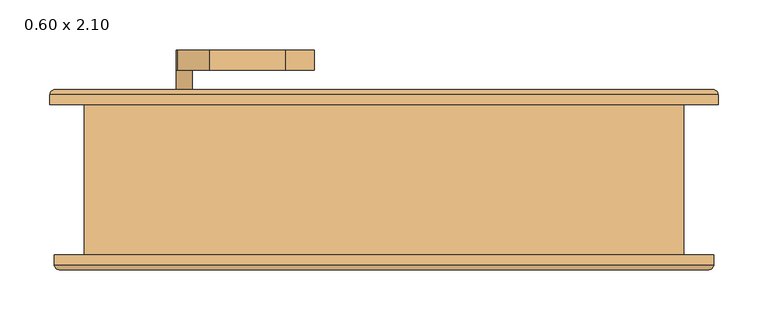
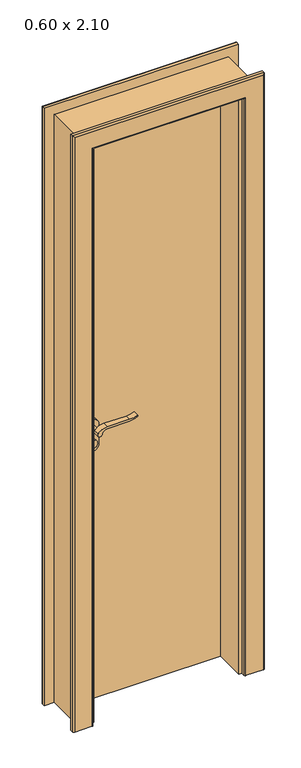
"""IFC4 building model written with IfcOpenShell, lengths in millimetres: door geometry, PORTA_DE_ABRIR_MADEIRA : 0.60 x 2.10."""

import ifcopenshell
import ifcopenshell.guid

model = None  # the IFC model being written
_history = None  # IfcOwnerHistory: only IFC2X3 demands one
_inside = {}  # id of a spatial element -> (the spatial element, [elements in it])
_under = {}  # id of a project, library or spatial element -> (it, [spatial elements below it])
_declared = {}  # id of a project -> (the project, [libraries it declares])
_typed = {}  # id of a type object -> (the type object, [elements of that type])
_made_of = {}  # id of a material, layer set ... -> (it, [elements and type objects made of it])


def new_model(schema):
    """Start an empty IFC model of exactly this schema.

    Asked for "IFC4X3", IfcOpenShell would pick the latest addendum, in which some entities
    have other attributes; the version numbers below select the first issue.
    IFC2X3 requires an IfcOwnerHistory on every rooted entity: one is made here for all.
    """
    global model, _history
    if schema == "IFC4X3":
        model = ifcopenshell.file(schema_version=(4, 3, 0, 0))
    else:
        model = ifcopenshell.file(schema=schema)
    _inside.clear()
    _under.clear()
    _declared.clear()
    _typed.clear()
    _made_of.clear()
    _history = None
    if model.schema == "IFC2X3":
        org = make("IfcOrganization", Name="unknown")
        user = make(
            "IfcPersonAndOrganization",
            ThePerson=make("IfcPerson", FamilyName="unknown"),
            TheOrganization=org,
        )
        app = make(
            "IfcApplication",
            ApplicationDeveloper=org,
            Version="unknown",
            ApplicationFullName="unknown",
            ApplicationIdentifier="unknown",
        )
        _history = make(
            "IfcOwnerHistory",
            OwningUser=user,
            OwningApplication=app,
            ChangeAction="ADDED",
            CreationDate=0,
        )
    return model


def make(cls, **values):
    """One entity of the class cls with the attributes given. An attribute that is None is left unset."""
    return model.create_entity(
        cls, **{name: value for name, value in values.items() if value is not None}
    )


def rooted(cls, **values):
    """An entity with a GlobalId (a new one), such as an element, a storey or a relation."""
    return make(cls, GlobalId=ifcopenshell.guid.new(), OwnerHistory=_history, **values)


def si_unit(unit_type, name, prefix=None):
    """IfcSIUnit, for example si_unit("LENGTHUNIT", "METRE", prefix="MILLI")."""
    return make("IfcSIUnit", UnitType=unit_type, Prefix=prefix, Name=name)


def assignment(units):
    """IfcUnitAssignment: the units of a project."""
    return None if units is None else make("IfcUnitAssignment", Units=units)


def point(xyz):
    """IfcCartesianPoint."""
    return None if xyz is None else make("IfcCartesianPoint", Coordinates=xyz)


def direction(xyz):
    """IfcDirection."""
    return None if xyz is None else make("IfcDirection", DirectionRatios=xyz)


def frame(location, z_axis=None, x_axis=None):
    """IfcAxis2Placement3D, a coordinate frame: its origin and axes. An axis left out is left unset."""
    return make(
        "IfcAxis2Placement3D",
        Location=point(location),
        Axis=direction(z_axis),
        RefDirection=direction(x_axis),
    )


def frame_2d(location, x_axis=None):
    """IfcAxis2Placement2D, a coordinate frame in the plane: its origin and x axis."""
    return make(
        "IfcAxis2Placement2D", Location=point(location), RefDirection=direction(x_axis)
    )


def origin():
    """The frame at (0, 0, 0) with its axes left unset."""
    return frame((0.0, 0.0, 0.0))


def origin_with_axes():
    """The frame at (0, 0, 0) with the z axis (0, 0, 1) and the x axis (1, 0, 0) written out."""
    return frame((0.0, 0.0, 0.0), z_axis=(0.0, 0.0, 1.0), x_axis=(1.0, 0.0, 0.0))


def place(relative_to, where):
    """IfcLocalPlacement: puts the frame where relative to a parent placement (None: the world)."""
    return make(
        "IfcLocalPlacement", PlacementRelTo=relative_to, RelativePlacement=where
    )


def context(
    kind, dimensions, precision=None, world=None, true_north=None, identifier=None
):
    """IfcGeometricRepresentationContext, for example the 3D "Model" context."""
    return make(
        "IfcGeometricRepresentationContext",
        ContextIdentifier=identifier,
        ContextType=kind,
        CoordinateSpaceDimension=dimensions,
        Precision=precision,
        WorldCoordinateSystem=world,
        TrueNorth=true_north,
    )


def project(units=None, contexts=None):
    """IfcProject with its units and contexts."""
    return rooted(
        "IfcProject",
        Name="project",
        RepresentationContexts=contexts,
        UnitsInContext=assignment(units),
    )


def spatial(cls, under=None, at=None, **own):
    """A site, building, storey or space (cls), placed at a placement, below another one or the project."""
    s = rooted(cls, ObjectPlacement=at, **own)
    if under is not None:
        _under.setdefault(under.id(), (under, []))[1].append(s)
    return s


def polyline(points):
    """IfcPolyline through the points."""
    return make("IfcPolyline", Points=[point(p) for p in points])


def circle_curve(where, radius):
    """IfcCircle in the frame where."""
    return make("IfcCircle", Position=where, Radius=radius)


def ellipse_curve(where, semi_axis1, semi_axis2):
    """IfcEllipse in the frame where."""
    return make(
        "IfcEllipse", Position=where, SemiAxis1=semi_axis1, SemiAxis2=semi_axis2
    )


def trimmed(basis, trim1, trim2, sense, master):
    """IfcTrimmedCurve: the piece of a basis curve between two trims."""
    return make(
        "IfcTrimmedCurve",
        BasisCurve=basis,
        Trim1=trim1,
        Trim2=trim2,
        SenseAgreement=sense,
        MasterRepresentation=master,
    )


def segment(curve, same_sense, transition):
    """IfcCompositeCurveSegment."""
    return make(
        "IfcCompositeCurveSegment",
        Transition=transition,
        SameSense=same_sense,
        ParentCurve=curve,
    )


def composite_curve(segments, self_intersect=None):
    """IfcCompositeCurve: segments joined end to end."""
    return make("IfcCompositeCurve", Segments=segments, SelfIntersect=self_intersect)


def outline(outer, holes=None, kind="AREA"):
    """IfcArbitraryClosedProfileDef: a profile drawn as a closed curve; with holes, ...WithVoids."""
    if holes is None:
        return make("IfcArbitraryClosedProfileDef", ProfileType=kind, OuterCurve=outer)
    return make(
        "IfcArbitraryProfileDefWithVoids",
        ProfileType=kind,
        OuterCurve=outer,
        InnerCurves=holes,
    )


def extrude(swept, where, along, depth):
    """IfcExtrudedAreaSolid: the profile swept, set in the frame where, extruded along a direction by depth."""
    return make(
        "IfcExtrudedAreaSolid",
        SweptArea=swept,
        Position=where,
        ExtrudedDirection=direction(along),
        Depth=depth,
    )


def faces_of(points, faces, orient=None, outer=None):
    """IfcFace entities. A face is a list of loops; a loop is a list of indices into points, from 0.

    orient and outer hold one flag for each loop. By default every Orientation is true, the
    first loop of a face is its IfcFaceOuterBound and the others are IfcFaceBound.
    """
    made = []
    for i, loops in enumerate(faces):
        bounds = []
        for j, loop in enumerate(loops):
            is_outer = j == 0 if outer is None else outer[i][j]
            bounds.append(
                make(
                    "IfcFaceOuterBound" if is_outer else "IfcFaceBound",
                    Bound=make("IfcPolyLoop", Polygon=[points[k] for k in loop]),
                    Orientation=True if orient is None else orient[i][j],
                )
            )
        made.append(make("IfcFace", Bounds=bounds))
    return made


def faceted_brep(points, faces, orient=None, outer=None, voids=None):
    """IfcFacetedBrep: a solid bounded by flat faces; with voids (closed shells), ...WithVoids."""
    shared = [point(p) for p in points]
    hull = make("IfcClosedShell", CfsFaces=faces_of(shared, faces, orient, outer))
    if voids is None:
        return make("IfcFacetedBrep", Outer=hull)
    return make(
        "IfcFacetedBrepWithVoids",
        Outer=hull,
        Voids=[
            make(cls, CfsFaces=faces_of(shared, fs, o, b)) for cls, fs, o, b in voids
        ],
    )


def shape(context_of_items, identifier, shape_type, items):
    """IfcShapeRepresentation: the items that make up one representation, for example the "Body"."""
    return make(
        "IfcShapeRepresentation",
        ContextOfItems=context_of_items,
        RepresentationIdentifier=identifier,
        RepresentationType=shape_type,
        Items=items,
    )


def source(mapping_origin, context_of_items, identifier, shape_type, items):
    """IfcRepresentationMap: a shape defined once, which mapped items show again and again."""
    return make(
        "IfcRepresentationMap",
        MappingOrigin=mapping_origin,
        MappedRepresentation=shape(context_of_items, identifier, shape_type, items),
    )


def transform(
    local_origin,
    x_axis=None,
    y_axis=None,
    z_axis=None,
    scale=None,
    scale2=None,
    scale3=None,
    uniform=True,
):
    """IfcCartesianTransformationOperator3D, or its non-uniform kind. x_axis, y_axis, z_axis: its Axis1, 2, 3."""
    if uniform:
        return make(
            "IfcCartesianTransformationOperator3D",
            Axis1=direction(x_axis),
            Axis2=direction(y_axis),
            LocalOrigin=point(local_origin),
            Scale=scale,
            Axis3=direction(z_axis),
        )
    return make(
        "IfcCartesianTransformationOperator3DnonUniform",
        Axis1=direction(x_axis),
        Axis2=direction(y_axis),
        LocalOrigin=point(local_origin),
        Scale=scale,
        Axis3=direction(z_axis),
        Scale2=scale2,
        Scale3=scale3,
    )


def mapped(mapping_source, mapping_target):
    """IfcMappedItem: shows the shape of a source again, moved by a transform."""
    return make(
        "IfcMappedItem", MappingSource=mapping_source, MappingTarget=mapping_target
    )


def made_of(thing, what):
    """Note that an element or type object is made of a material, layer set ...; save() writes the relation."""
    if what is not None:
        _made_of.setdefault(what.id(), (what, []))[1].append(thing)
    return thing


def element(
    cls,
    number,
    at=None,
    inside=None,
    cuts=None,
    type_object=None,
    material=None,
    context=None,
    identifier="Body",
    shape_type=None,
    held_by="IfcProductDefinitionShape",
    body=None,
    shapes=None,
    **own,
):
    """One element of the class cls, such as IfcWall. Its Tag is "e" and its number.

    at: its placement. inside: the storey or other place that contains it. cuts: it is an
    opening in that element (IfcRelVoidsElement). A single representation is given by context,
    identifier, shape_type and body (its items); several are given by shapes. held_by: the class
    of the entity that holds the representations. save() writes the other relations.
    """
    e = rooted(cls, Tag="e%d" % number, ObjectPlacement=at, **own)
    if body is not None:
        shapes = [shape(context, identifier, shape_type, body)]
    if shapes is not None:
        e.Representation = make(held_by, Representations=shapes)
    if inside is not None:
        _inside.setdefault(inside.id(), (inside, []))[1].append(e)
    if cuts is not None:
        rooted(
            "IfcRelVoidsElement", RelatingBuildingElement=cuts, RelatedOpeningElement=e
        )
    if type_object is not None:
        _typed.setdefault(type_object.id(), (type_object, []))[1].append(e)
    return made_of(e, material)


def aggregate(whole, parts):
    """IfcRelAggregates: a whole, such as a stair, and the parts it consists of."""
    return rooted("IfcRelAggregates", RelatingObject=whole, RelatedObjects=parts)


def save(model, path):
    """Write the relations noted so far, then the file.

    IfcRelAggregates (storeys below a building ...), IfcRelContainedInSpatialStructure (elements
    in a storey), IfcRelDefinesByType, IfcRelAssociatesMaterial and IfcRelDeclares: one each for
    every whole, place, type object, material and project.
    """
    for whole, parts in _under.values():
        aggregate(whole, parts)
    for where, things in _inside.values():
        rooted(
            "IfcRelContainedInSpatialStructure",
            RelatedElements=things,
            RelatingStructure=where,
        )
    for kind, things in _typed.values():
        rooted("IfcRelDefinesByType", RelatedObjects=things, RelatingType=kind)
    for what, things in _made_of.values():
        rooted("IfcRelAssociatesMaterial", RelatedObjects=things, RelatingMaterial=what)
    for by, libraries in _declared.values():
        rooted("IfcRelDeclares", RelatingContext=by, RelatedDefinitions=libraries)
    model.write(path)


def plane_surface(at):
    """IfcPlane: the flat surface through the origin of the frame at, square to its z axis."""
    return make("IfcPlane", Position=at)


def cylinder_surface(at, radius):
    """IfcCylindricalSurface: all points at the distance radius from the z axis of the frame at."""
    return make("IfcCylindricalSurface", Position=at, Radius=radius)


def advanced_brep(points, edges, surfaces, faces):
    """IfcAdvancedBrep: a solid bounded by faces that lie on surfaces and meet in shared edges.

    An edge is (start, end): straight between two places in points (the first is 0);
    or (start, end, curve); or (start, end, curve, False) where it runs against its curve.
    A face is (place in surfaces, loops), or (place, loops, False) where it looks against
    its surface's normal. A loop lists edges by number (the first is 1), with a minus sign
    where the edge is run from its end to its start. The first loop is the outer one.
    """
    corners = [point(p) for p in points]
    vertices = [make("IfcVertexPoint", VertexGeometry=c) for c in corners]
    made = []
    for start, end, *more in edges:
        made.append(
            make(
                "IfcEdgeCurve",
                EdgeStart=vertices[start],
                EdgeEnd=vertices[end],
                EdgeGeometry=more[0] if more else make("IfcPolyline", Points=[corners[start], corners[end]]),
                SameSense=more[1] if len(more) > 1 else True,
            )
        )
    hull = []
    for where, loops, *sense in faces:
        bounds = []
        for j, loop in enumerate(loops):
            ring = [make("IfcOrientedEdge", EdgeElement=made[abs(k) - 1], Orientation=k > 0) for k in loop]
            bounds.append(
                make(
                    "IfcFaceOuterBound" if j == 0 else "IfcFaceBound",
                    Bound=make("IfcEdgeLoop", EdgeList=ring),
                    Orientation=True,
                )
            )
        hull.append(make("IfcAdvancedFace", Bounds=bounds, FaceSurface=surfaces[where], SameSense=sense[0] if sense else True))
    return make("IfcAdvancedBrep", Outer=make("IfcClosedShell", CfsFaces=hull))


def door_0_60_x_2_10_4441030f(model_context):
    return source(origin(), model_context, "Body", "SolidModel", [
        extrude(outline(composite_curve([segment(trimmed(circle_curve(frame_2d((940.0, -200.0)), 15.0), [point((940.0, -185.0))], [point((940.0, -215.0))], False, "CARTESIAN"), True, "CONTINUOUS"), segment(trimmed(circle_curve(frame_2d((940.0, -200.0)), 15.0), [point((940.0, -215.0))], [point((940.0, -185.0))], False, "CARTESIAN"), True, "CONTINUOUS")], self_intersect=False)), frame((0.0, 15.0, 0.0), z_axis=(0.0, 1.0, 0.0), x_axis=(0.0, 0.0, 1.0)), (0.0, 0.0, 1.0), 10.0),
        extrude(outline(composite_curve([segment(trimmed(circle_curve(frame_2d((940.0, -200.0)), 15.0), [point((940.0, -185.0))], [point((940.0, -215.0))], False, "CARTESIAN"), True, "CONTINUOUS"), segment(trimmed(circle_curve(frame_2d((940.0, -200.0)), 15.0), [point((940.0, -215.0))], [point((940.0, -185.0))], False, "CARTESIAN"), True, "CONTINUOUS")], self_intersect=False)), frame((0.0, 80.0, 0.0), z_axis=(0.0, 1.0, 0.0), x_axis=(0.0, 0.0, 1.0)), (0.0, 0.0, 1.0), 10.0),
        extrude(outline(composite_curve([segment(trimmed(circle_curve(frame_2d((1000.0, -200.0)), 8.0), [point((1004.6523287, -206.5081363))], [point((1000.0, -192.0))], False, "CARTESIAN"), True, "CONTINUOUS"), segment(trimmed(circle_curve(frame_2d((994.8738613, -174.6138099)), 18.1261387), [point((1000.0, -192.0))], [point((1013.0, -174.6138099))], True, "CARTESIAN"), True, "CONTINUOUS"), segment(polyline([(1013.0, -174.6138099), (1013.0, -98.3564091)]), True, "CONTINUOUS"), segment(trimmed(circle_curve(frame_2d((1072.2709207, -101.9396612)), 59.3791355), [point((1013.0, -98.3564091))], [point((1022.2135558, -70.0))], False, "CARTESIAN"), True, "CONTINUOUS"), segment(polyline([(1022.2135558, -70.0), (1025.0, -70.0)]), True, "CONTINUOUS"), segment(trimmed(circle_curve(frame_2d((1103.2850638, -98.4227909)), 83.2850902), [point((1025.0, -70.0))], [point((1020.0, -98.3564091))], True, "CARTESIAN"), True, "CONTINUOUS"), segment(polyline([(1020.0, -98.3564091), (1020.0, -174.6325667)]), True, "CONTINUOUS"), segment(trimmed(circle_curve(frame_2d((982.7555521, -176.3324871)), 37.2832219), [point((1020.0, -174.6325667))], [point((1004.6523287, -206.5081363))], False, "CARTESIAN"), True, "CONTINUOUS")], self_intersect=False)), frame((0.0, -25.0, 0.0), z_axis=(0.0, 1.0, 0.0), x_axis=(0.0, 0.0, 1.0)), (0.0, 0.0, 1.0), 20.0),
        extrude(outline(composite_curve([segment(trimmed(circle_curve(frame_2d((994.8738682, -174.6138122)), 18.1261318), [point((999.9999903, -192.0))], [point((1013.0, -174.6138122))], True, "CARTESIAN"), True, "CONTINUOUS"), segment(polyline([(1013.0, -174.6138122), (1013.0, -98.3564091)]), True, "CONTINUOUS"), segment(trimmed(circle_curve(frame_2d((1072.2709207, -101.9396612)), 59.3791355), [point((1013.0, -98.3564091))], [point((1022.2135558, -70.0))], False, "CARTESIAN"), True, "CONTINUOUS"), segment(polyline([(1022.2135558, -70.0), (1025.0, -70.0)]), True, "CONTINUOUS"), segment(trimmed(circle_curve(frame_2d((1103.2850638, -98.4227909)), 83.2850902), [point((1025.0, -70.0))], [point((1020.0, -98.3564091))], True, "CARTESIAN"), True, "CONTINUOUS"), segment(polyline([(1020.0, -98.3564091), (1020.0, -174.6325667)]), True, "CONTINUOUS"), segment(trimmed(circle_curve(frame_2d((982.7555521, -176.3324871)), 37.2832219), [point((1020.0, -174.6325667))], [point((1004.6523287, -206.5081363))], False, "CARTESIAN"), True, "CONTINUOUS"), segment(trimmed(circle_curve(frame_2d((1000.0, -200.0)), 8.0), [point((1004.6523287, -206.5081363))], [point((999.9999903, -192.0))], False, "CARTESIAN"), True, "CONTINUOUS")], self_intersect=False)), frame((0.0, 110.0, 0.0), z_axis=(0.0, 1.0, 0.0), x_axis=(0.0, 0.0, 1.0)), (0.0, 0.0, 1.0), 20.0),
        extrude(outline(composite_curve([segment(trimmed(circle_curve(frame_2d((1000.0, -200.0)), 8.0), [point((1000.0, -192.0))], [point((1000.0, -208.0))], False, "CARTESIAN"), True, "CONTINUOUS"), segment(trimmed(circle_curve(frame_2d((1000.0, -200.0)), 8.0), [point((1000.0, -208.0))], [point((1000.0, -192.0))], False, "CARTESIAN"), True, "CONTINUOUS")], self_intersect=False)), frame((0.0, -5.0, 0.0), z_axis=(0.0, 1.0, 0.0), x_axis=(0.0, 0.0, 1.0)), (0.0, 0.0, 1.0), 30.0),
        extrude(outline(composite_curve([segment(trimmed(circle_curve(frame_2d((1000.0, -200.0)), 8.0), [point((1000.0, -192.0))], [point((1000.0, -208.0))], False, "CARTESIAN"), True, "CONTINUOUS"), segment(trimmed(circle_curve(frame_2d((1000.0, -200.0)), 8.0), [point((1000.0, -208.0))], [point((1000.0, -192.0))], False, "CARTESIAN"), True, "CONTINUOUS")], self_intersect=False)), frame((0.0, 80.0, 0.0), z_axis=(0.0, 1.0, 0.0), x_axis=(0.0, 0.0, 1.0)), (0.0, 0.0, 1.0), 30.0),
        extrude(outline(composite_curve([segment(trimmed(circle_curve(frame_2d((930.0, -200.0)), 25.0), [point((930.0, -225.0))], [point((930.0, -175.0))], False, "CARTESIAN"), True, "CONTINUOUS"), segment(polyline([(930.0, -175.0), (1000.0, -175.0)]), True, "CONTINUOUS"), segment(trimmed(circle_curve(frame_2d((1000.0, -200.0)), 25.0), [point((1000.0, -175.0))], [point((1000.0, -225.0))], False, "CARTESIAN"), True, "CONTINUOUS"), segment(polyline([(1000.0, -225.0), (930.0, -225.0)]), True, "CONTINUOUS")], self_intersect=False)), frame((0.0, 25.0, 0.0), z_axis=(0.0, 1.0, 0.0), x_axis=(0.0, 0.0, 1.0)), (0.0, 0.0, 1.0), 10.0),
        extrude(outline(composite_curve([segment(trimmed(circle_curve(frame_2d((930.0, -200.0)), 25.0), [point((930.0, -225.0))], [point((930.0, -175.0))], False, "CARTESIAN"), True, "CONTINUOUS"), segment(polyline([(930.0, -175.0), (1000.0, -175.0)]), True, "CONTINUOUS"), segment(trimmed(circle_curve(frame_2d((1000.0, -200.0)), 25.0), [point((1000.0, -175.0))], [point((1000.0, -225.0))], False, "CARTESIAN"), True, "CONTINUOUS"), segment(polyline([(1000.0, -225.0), (930.0, -225.0)]), True, "CONTINUOUS")], self_intersect=False)), frame((0.0, 70.0, 0.0), z_axis=(0.0, 1.0, 0.0), x_axis=(0.0, 0.0, 1.0)), (0.0, 0.0, 1.0), 10.0),
        faceted_brep([(-260.0, 35.0, 0.0), (-250.0, 35.0, 0.0), (-250.0, -75.0, 0.0), (-300.0, -75.0, 0.0), (-300.0, 75.0, 0.0), (-260.0, 75.0, 0.0), (-260.0, 75.0, 2100.0), (-260.0, 35.0, 2100.0), (-300.0, 75.0, 2140.0), (300.0, 75.0, 2140.0), (300.0, 75.0, 0.0), (260.0, 75.0, 0.0), (260.0, 75.0, 2100.0), (-300.0, -75.0, 2140.0), (-250.0, -75.0, 2090.0), (250.0, -75.0, 2090.0), (250.0, -75.0, 0.0), (300.0, -75.0, 0.0), (300.0, -75.0, 2140.0), (-250.0, 35.0, 2090.0), (260.0, 35.0, 2100.0), (260.0, 35.0, 0.0), (250.0, 35.0, 0.0), (250.0, 35.0, 2090.0)], [[[0, 1, 2, 3, 4, 5]], [[5, 6, 7, 0]], [[4, 8, 9, 10, 11, 12, 6, 5]], [[3, 13, 8, 4]], [[2, 14, 15, 16, 17, 18, 13, 3]], [[1, 19, 14, 2]], [[0, 7, 20, 21, 22, 23, 19, 1]], [[23, 22, 16, 15]], [[21, 11, 10, 17, 16, 22]], [[12, 11, 21, 20]], [[18, 17, 10, 9]], [[13, 18, 9, 8]], [[19, 23, 15, 14]], [[6, 12, 20, 7]]]),
        advanced_brep(
        [(-330.0, -75.3, 0.0), (-260.0, -75.3, 0.0), (-260.0, -85.3, 0.0), (-265.0, -90.3, 0.0), (-325.0, -90.3, 0.0), (-330.0, -85.3, 0.0), (-330.0, -85.3, 2170.0), (-330.0, -75.3, 2170.0), (-325.0, -90.3, 2165.0), (-265.0, -90.3, 2105.0), (265.0, -90.3, 2105.0), (265.0, -90.3, 0.0), (325.0, -90.3, 0.0), (325.0, -90.3, 2165.0), (-260.0, -85.3, 2100.0), (-260.0, -75.3, 2100.0), (330.0, -75.3, 2170.0), (330.0, -75.3, 0.0), (260.0, -75.3, 0.0), (260.0, -75.3, 2100.0), (330.0, -85.3, 0.0), (260.0, -85.3, 0.0), (260.0, -85.3, 2100.0), (330.0, -85.3, 2170.0)],
        [
            (0, 1),
            (1, 2),
            (2, 3, circle_curve(frame((-265.0, -85.3, 0.0), z_axis=(0.0, 0.0, -1.0), x_axis=(-1.0, 0.0, 0.0)), 5.0)),
            (3, 4),
            (4, 5, circle_curve(frame((-325.0, -85.3, 0.0), z_axis=(0.0, 0.0, -1.0), x_axis=(-1.0, 0.0, 0.0)), 5.0)),
            (5, 0),
            (5, 6),
            (6, 7),
            (7, 0),
            (4, 8),
            (8, 6, ellipse_curve(frame((-325.0, -85.3, 2165.0), z_axis=(-0.7071067811865475, 0.0, -0.7071067811865475), x_axis=(0.7071067811865474, 0.0, -0.7071067811865476)), 7.0710678, 5.0)),
            (3, 9),
            (9, 10),
            (10, 11),
            (11, 12),
            (12, 13),
            (13, 8),
            (2, 14),
            (14, 9, ellipse_curve(frame((-265.0, -85.3, 2105.0), z_axis=(-0.7071067811865475, 0.0, -0.7071067811865475), x_axis=(0.7071067811865474, 0.0, -0.7071067811865476)), 7.0710678, 5.0)),
            (1, 15),
            (15, 14),
            (7, 16),
            (16, 17),
            (17, 18),
            (18, 19),
            (19, 15),
            (17, 20),
            (20, 12, circle_curve(frame((325.0, -85.3, 0.0), z_axis=(0.0, 0.0, -1.0), x_axis=(1.0, 0.0, 0.0)), 5.0)),
            (11, 21, circle_curve(frame((265.0, -85.3, 0.0), z_axis=(0.0, 0.0, -1.0), x_axis=(1.0, 0.0, 0.0)), 5.0)),
            (21, 18),
            (21, 22),
            (22, 19),
            (10, 22, ellipse_curve(frame((265.0, -85.3, 2105.0), z_axis=(0.7071067811865475, 0.0, -0.7071067811865475), x_axis=(0.7071067811865474, 0.0, 0.7071067811865476)), 7.0710678, 5.0)),
            (20, 23),
            (23, 13, ellipse_curve(frame((325.0, -85.3, 2165.0), z_axis=(0.7071067811865475, 0.0, -0.7071067811865475), x_axis=(0.7071067811865474, 0.0, 0.7071067811865476)), 7.0710678, 5.0)),
            (16, 23),
            (6, 23),
            (22, 14),
        ],
        [
            plane_surface(frame((-300.0, 75.0, 0.0), z_axis=(0.0, 0.0, -1.0), x_axis=(0.0, 1.0, 0.0))),
            plane_surface(frame((-330.0, -75.3, 0.0), z_axis=(-1.0, 0.0, 0.0), x_axis=(0.0, 0.0, 1.0))),
            cylinder_surface(frame((-325.0, -85.3, 0.0), z_axis=(0.0, 0.0, -1.0), x_axis=(-1.0, 0.0, 0.0)), 5.0),
            plane_surface(frame((-325.0, -90.3, 0.0), z_axis=(0.0, -1.0, 0.0), x_axis=(0.0, 0.0, 1.0))),
            cylinder_surface(frame((-265.0, -85.3, 0.0), z_axis=(0.0, 0.0, -1.0), x_axis=(-1.0, 0.0, 0.0)), 5.0),
            plane_surface(frame((-260.0, -85.3, 0.0), z_axis=(1.0, 0.0, 0.0), x_axis=(0.0, 0.0, 1.0))),
            plane_surface(frame((-260.0, -75.3, 0.0), z_axis=(0.0, 1.0, 0.0), x_axis=(0.0, 0.0, 1.0))),
            plane_surface(frame((300.0, 75.0, 0.0), z_axis=(0.0, 0.0, -1.0), x_axis=(0.0, 1.0, 0.0))),
            plane_surface(frame((260.0, -85.3, 2100.0), z_axis=(-1.0, 0.0, 0.0), x_axis=(0.0, 0.0, -1.0))),
            cylinder_surface(frame((265.0, -85.3, 2140.0), z_axis=(0.0, 0.0, 1.0), x_axis=(1.0, 0.0, 0.0)), 5.0),
            cylinder_surface(frame((325.0, -85.3, 2140.0), z_axis=(0.0, 0.0, 1.0), x_axis=(1.0, 0.0, 0.0)), 5.0),
            plane_surface(frame((330.0, -75.3, 2170.0), z_axis=(1.0, 0.0, 0.0), x_axis=(0.0, 0.0, -1.0))),
            plane_surface(frame((-330.0, -75.3, 2170.0), z_axis=(0.0, 0.0, 1.0), x_axis=(1.0, 0.0, 0.0))),
            plane_surface(frame((-260.0, -85.3, 2100.0), z_axis=(0.0, 0.0, -1.0), x_axis=(1.0, 0.0, 0.0))),
            cylinder_surface(frame((-300.0, -85.3, 2165.0), z_axis=(-1.0, 0.0, 0.0), x_axis=(0.0, 0.0, 1.0)), 5.0),
            cylinder_surface(frame((-300.0, -85.3, 2105.0), z_axis=(-1.0, 0.0, 0.0), x_axis=(0.0, 0.0, 1.0)), 5.0),
        ],
        [
            (0, [[1, 2, 3, 4, 5, 6]]),
            (1, [[7, 8, 9, -6]]),
            (2, [[10, 11, -7, -5]]),
            (3, [[12, 13, 14, 15, 16, 17, -10, -4]]),
            (4, [[18, 19, -12, -3]]),
            (5, [[20, 21, -18, -2]]),
            (6, [[-9, 22, 23, 24, 25, 26, -20, -1]]),
            (7, [[27, 28, -15, 29, 30, -24]]),
            (8, [[-25, -30, 31, 32]]),
            (9, [[-31, -29, -14, 33]]),
            (10, [[-16, -28, 34, 35]]),
            (11, [[-34, -27, -23, 36]]),
            (12, [[37, -36, -22, -8]]),
            (13, [[-26, -32, 38, -21]]),
            (14, [[-17, -35, -37, -11]]),
            (15, [[-38, -33, -13, -19]]),
        ],
    ),
        advanced_brep(
        [(-329.3155593, 90.2647517, 0.0), (-269.3155593, 90.2647517, 0.0), (-264.3155593, 85.2647517, 0.0), (-264.3155593, 75.2647517, 0.0), (-334.3155593, 75.2647517, 0.0), (-334.3155593, 85.2647517, 0.0), (-334.3155593, 85.2647517, 2174.3155593), (-329.3155593, 90.2647517, 2169.3155593), (-334.3155593, 75.2647517, 2174.3155593), (-264.3155593, 75.2647517, 2104.3155593), (264.3155593, 75.2647517, 2104.3155593), (264.3155593, 75.2647517, 0.0), (334.3155593, 75.2647517, 0.0), (334.3155593, 75.2647517, 2174.3155593), (-264.3155593, 85.2647517, 2104.3155593), (-269.3155593, 90.2647517, 2109.3155593), (329.3155593, 90.2647517, 2169.3155593), (329.3155593, 90.2647517, 0.0), (269.3155593, 90.2647517, 0.0), (269.3155593, 90.2647517, 2109.3155593), (334.3155593, 85.2647517, 0.0), (264.3155593, 85.2647517, 0.0), (264.3155593, 85.2647517, 2104.3155593), (334.3155593, 85.2647517, 2174.3155593)],
        [
            (0, 1),
            (1, 2, circle_curve(frame((-269.3155593, 85.2647517, 0.0), z_axis=(0.0, 0.0, -1.0), x_axis=(-1.0, 0.0, 0.0)), 5.0)),
            (2, 3),
            (3, 4),
            (4, 5),
            (5, 0, circle_curve(frame((-329.3155593, 85.2647517, 0.0), z_axis=(0.0, 0.0, -1.0), x_axis=(-1.0, 0.0, 0.0)), 5.0)),
            (5, 6),
            (6, 7, ellipse_curve(frame((-329.3155593, 85.2647517, 2169.3155593), z_axis=(-0.7071067811865475, 0.0, -0.7071067811865475), x_axis=(0.7071067811865474, 0.0, -0.7071067811865476)), 7.0710678, 5.0)),
            (7, 0),
            (4, 8),
            (8, 6),
            (3, 9),
            (9, 10),
            (10, 11),
            (11, 12),
            (12, 13),
            (13, 8),
            (2, 14),
            (14, 9),
            (1, 15),
            (15, 14, ellipse_curve(frame((-269.3155593, 85.2647517, 2109.3155593), z_axis=(-0.7071067811865475, 0.0, -0.7071067811865475), x_axis=(0.7071067811865474, 0.0, -0.7071067811865476)), 7.0710678, 5.0)),
            (7, 16),
            (16, 17),
            (17, 18),
            (18, 19),
            (19, 15),
            (17, 20, circle_curve(frame((329.3155593, 85.2647517, 0.0), z_axis=(0.0, 0.0, -1.0), x_axis=(1.0, 0.0, 0.0)), 5.0)),
            (20, 12),
            (11, 21),
            (21, 18, circle_curve(frame((269.3155593, 85.2647517, 0.0), z_axis=(0.0, 0.0, -1.0), x_axis=(1.0, 0.0, 0.0)), 5.0)),
            (21, 22),
            (22, 19, ellipse_curve(frame((269.3155593, 85.2647517, 2109.3155593), z_axis=(0.7071067811865475, 0.0, -0.7071067811865475), x_axis=(0.7071067811865474, 0.0, 0.7071067811865476)), 7.0710678, 5.0)),
            (10, 22),
            (20, 23),
            (23, 13),
            (16, 23, ellipse_curve(frame((329.3155593, 85.2647517, 2169.3155593), z_axis=(0.7071067811865475, 0.0, -0.7071067811865475), x_axis=(0.7071067811865474, 0.0, 0.7071067811865476)), 7.0710678, 5.0)),
            (23, 6),
            (14, 22),
        ],
        [
            plane_surface(frame((-300.0, 75.0, 0.0), z_axis=(0.0, 0.0, -1.0), x_axis=(0.0, 1.0, 0.0))),
            cylinder_surface(frame((-329.3155593, 85.2647517, 0.0), z_axis=(0.0, 0.0, -1.0), x_axis=(-1.0, 0.0, 0.0)), 5.0),
            plane_surface(frame((-334.3155593, 85.2647517, 0.0), z_axis=(-1.0, 0.0, 0.0), x_axis=(0.0, 0.0, 1.0))),
            plane_surface(frame((-334.3155593, 75.2647517, 0.0), z_axis=(0.0, -1.0, 0.0), x_axis=(0.0, 0.0, 1.0))),
            plane_surface(frame((-264.3155593, 75.2647517, 0.0), z_axis=(1.0, 0.0, 0.0), x_axis=(0.0, 0.0, 1.0))),
            cylinder_surface(frame((-269.3155593, 85.2647517, 0.0), z_axis=(0.0, 0.0, -1.0), x_axis=(-1.0, 0.0, 0.0)), 5.0),
            plane_surface(frame((-269.3155593, 90.2647517, 0.0), z_axis=(0.0, 1.0, 0.0), x_axis=(0.0, 0.0, 1.0))),
            plane_surface(frame((300.0, 75.0, 0.0), z_axis=(0.0, 0.0, -1.0), x_axis=(0.0, 1.0, 0.0))),
            cylinder_surface(frame((269.3155593, 85.2647517, 2140.0), z_axis=(0.0, 0.0, 1.0), x_axis=(1.0, 0.0, 0.0)), 5.0),
            plane_surface(frame((264.3155593, 75.2647517, 2104.3155593), z_axis=(-1.0, 0.0, 0.0), x_axis=(0.0, 0.0, -1.0))),
            plane_surface(frame((334.3155593, 85.2647517, 2174.3155593), z_axis=(1.0, 0.0, 0.0), x_axis=(0.0, 0.0, -1.0))),
            cylinder_surface(frame((329.3155593, 85.2647517, 2140.0), z_axis=(0.0, 0.0, 1.0), x_axis=(1.0, 0.0, 0.0)), 5.0),
            plane_surface(frame((-334.3155593, 85.2647517, 2174.3155593), z_axis=(0.0, 0.0, 1.0), x_axis=(1.0, 0.0, 0.0))),
            plane_surface(frame((-264.3155593, 75.2647517, 2104.3155593), z_axis=(0.0, 0.0, -1.0), x_axis=(1.0, 0.0, 0.0))),
            cylinder_surface(frame((-300.0, 85.2647517, 2169.3155593), z_axis=(-1.0, 0.0, 0.0), x_axis=(0.0, 0.0, 1.0)), 5.0),
            cylinder_surface(frame((-300.0, 85.2647517, 2109.3155593), z_axis=(-1.0, 0.0, 0.0), x_axis=(0.0, 0.0, 1.0)), 5.0),
        ],
        [
            (0, [[1, 2, 3, 4, 5, 6]]),
            (1, [[7, 8, 9, -6]]),
            (2, [[10, 11, -7, -5]]),
            (3, [[12, 13, 14, 15, 16, 17, -10, -4]]),
            (4, [[18, 19, -12, -3]]),
            (5, [[20, 21, -18, -2]]),
            (6, [[-9, 22, 23, 24, 25, 26, -20, -1]]),
            (7, [[27, 28, -15, 29, 30, -24]]),
            (8, [[-25, -30, 31, 32]]),
            (9, [[-31, -29, -14, 33]]),
            (10, [[-16, -28, 34, 35]]),
            (11, [[-34, -27, -23, 36]]),
            (12, [[-17, -35, 37, -11]]),
            (13, [[38, -33, -13, -19]]),
            (14, [[-37, -36, -22, -8]]),
            (15, [[-26, -32, -38, -21]]),
        ],
    ),
        extrude(outline(polyline([(260.0, 70.0), (260.0, 35.0), (-260.0, 35.0), (-260.0, 70.0), (260.0, 70.0)])), origin_with_axes(), (0.0, 0.0, 1.0), 2100.0),
    ])


if __name__ == "__main__":
    model = new_model("IFC4")
    model_context = context("Model", 3, world=origin())
    ifc_project = project(units=[si_unit("LENGTHUNIT", "METRE", prefix="MILLI")], contexts=[model_context])
    site = spatial("IfcSite", under=ifc_project)
    building = spatial("IfcBuilding", under=site)
    placement = place(None, origin())
    door_0_60_x_2_10_shape = door_0_60_x_2_10_4441030f(model_context)
    element("IfcDoor", 1, ObjectType="PORTA_DE_ABRIR_MADEIRA : 0.60 x 2.10", at=placement, inside=building, context=model_context, shape_type="MappedRepresentation", body=[
        mapped(door_0_60_x_2_10_shape, transform((0.0, 0.0, 0.0), x_axis=(1.0, 0.0, 0.0), y_axis=(0.0, 1.0, 0.0), z_axis=(0.0, 0.0, 1.0))),
    ])
    save(model, "model.ifc")

# Revit data of these elements
# Type "PORTA_DE_ABRIR_MADEIRA : 0.60 x 2.10"
#   Type Mark = "PV2"
#   Analytic Construction = "<Nenhum>"
#   Rough Width = 0.60 m
#   Projeção da estrutura externa = 0.025 m
#   Projeção da estrutura interna = 0.025 m
#   Largura da estrutura = 0.075 m
#   Rough Height = 2.15 m
#   Height = 2.10 m
#   Width = 0.70 m
#   Soleira [instance default] = no
#   Material do batente = .BATENTE E GUARNIÇÃO
#   Material da maçaneta = .AÇO INOXIDÁVEL ESCOVADO
#   Material da folha da porta = .FOLHA DA PORTA
#   Material da Soleira [instance default] = none
#   Function = (empty or 0)
#   Wall Closure = (empty or 0)
# Element 1 (IfcDoor, "PORTA_DE_ABRIR_MADEIRA : 0.60 x 2.10")
#   Materials on its faces: ".AÇO INOXIDÁVEL ESCOVADO", ".BATENTE E GUARNIÇÃO", ".FOLHA DA PORTA"
# Materials
#   ".BATENTE E GUARNIÇÃO": class "Madeira", colour RGB 215 186 156, transparency 0, Cost = 0
#   ".AÇO INOXIDÁVEL ESCOVADO": class "Metal", colour RGB 189 187 185, transparency 0, Description = "Stainless Steel 18/8, brushed finish", Cost = 0
#   ".FOLHA DA PORTA": class "Madeira", colour RGB 148 119 91, transparency 0, Cost = 0
